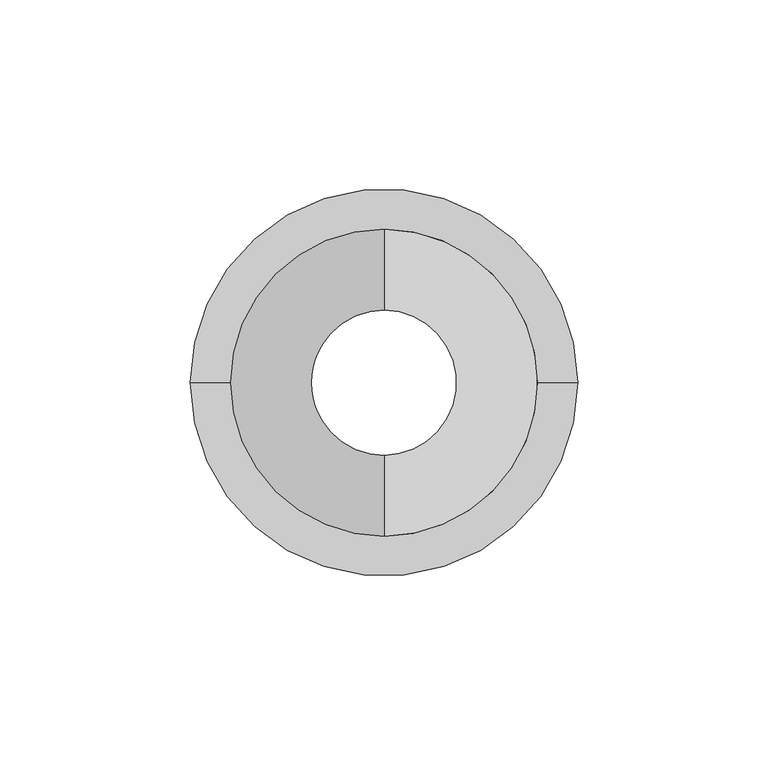
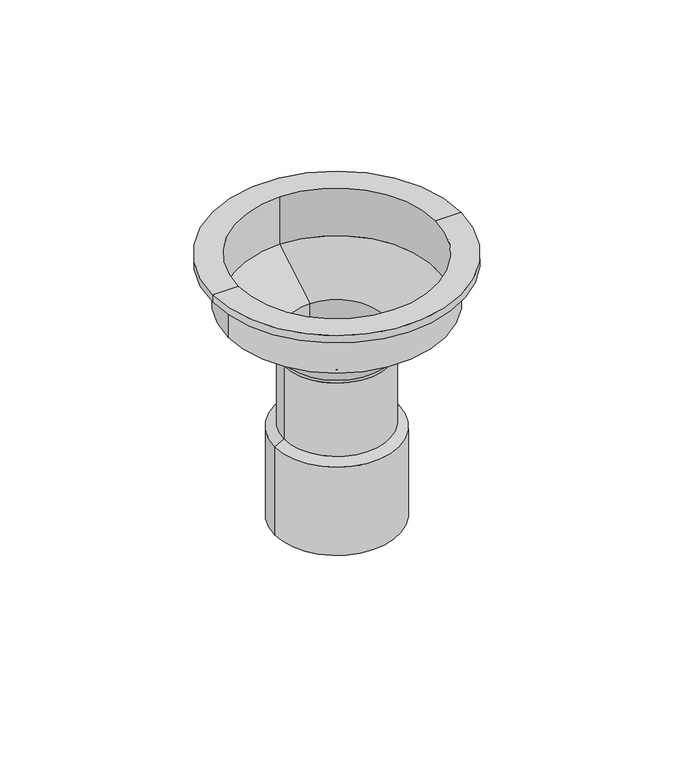
"""IFC4 building model written with IfcOpenShell, lengths in millimetres: proxy geometry, QF_BasketDrain_T&S Brass : QF_BasketDrain_T&S Brass."""

from ifc_helpers import new_model, si_unit, point, frame, origin, place, context, project, spatial, polyline, circle_curve, ellipse_curve, trimmed, source, transform, mapped, element, save
from ifc_brep_helpers import plane_surface, cylinder_surface, revolved_surface, advanced_brep


def specialty_equipment_44dcb793(model_context):
    return source(origin(), model_context, "Body", "AdvancedBrep", [
        advanced_brep(
        [(-25.4, -101.6, 449.2625), (25.4, -101.6, 449.2625), (19.05, -101.6, 449.2625), (0.0, -82.55, 449.2625), (-19.05, -101.6, 449.2625), (0.0, -120.65, 449.2625), (50.8, -101.6, 561.975), (-50.8, -101.6, 561.975), (-40.3518144, -101.6, 561.975), (0.0, -61.2481856, 561.975), (40.3518144, -101.6, 561.975), (0.0, -141.9518144, 561.975), (50.8, -101.6, 558.8), (-50.8, -101.6, 558.8), (44.45, -101.6, 558.8), (-44.45, -101.6, 558.8), (44.45, -101.6, 541.3375), (-44.45, -101.6, 541.3375), (22.253509, -101.6, 522.7124326), (-22.253509, -101.6, 522.7124326), (21.5046095, -101.6, 520.9369046), (-21.5046095, -101.6, 520.9369046), (21.5046095, -101.6, 489.3101953), (-21.5046095, -101.6, 489.3101953), (25.4, -101.6, 487.3625), (-25.4, -101.6, 487.3625), (0.0, -82.55, 528.6629098), (0.0, -120.65, 528.6629098), (0.0, -141.9518144, 541.3375), (0.0, -61.2481856, 541.3375)],
        [
            (0, 1, circle_curve(frame((0.0, -101.6, 449.2625), z_axis=(0.0, 0.0, -1.0), x_axis=(-1.0, 0.0, 0.0)), 25.4)),
            (1, 2),
            (2, 3, circle_curve(frame((0.0, -101.6, 449.2625), z_axis=(0.0, 0.0, 1.0), x_axis=(0.0, 1.0, 0.0)), 19.05)),
            (3, 4, circle_curve(frame((0.0, -101.6, 449.2625), z_axis=(0.0, 0.0, 1.0), x_axis=(0.0, 1.0, 0.0)), 19.05)),
            (4, 0),
            (1, 0, circle_curve(frame((0.0, -101.6, 449.2625), z_axis=(0.0, 0.0, -1.0), x_axis=(-1.0, 0.0, 0.0)), 25.4)),
            (4, 5, circle_curve(frame((0.0, -101.6, 449.2625), z_axis=(0.0, 0.0, 1.0), x_axis=(0.0, 1.0, 0.0)), 19.05)),
            (5, 2, circle_curve(frame((0.0, -101.6, 449.2625), z_axis=(0.0, 0.0, 1.0), x_axis=(0.0, 1.0, 0.0)), 19.05)),
            (6, 7, circle_curve(frame((0.0, -101.6, 561.975), z_axis=(0.0, 0.0, 1.0), x_axis=(-1.0, 0.0, 0.0)), 50.8)),
            (7, 8),
            (8, 9, circle_curve(frame((0.0, -101.6, 561.975), z_axis=(0.0, 0.0, -1.0), x_axis=(0.0, 1.0, 0.0)), 40.3518144)),
            (9, 10, circle_curve(frame((0.0, -101.6, 561.975), z_axis=(0.0, 0.0, -1.0), x_axis=(0.0, 1.0, 0.0)), 40.3518144)),
            (10, 6),
            (7, 6, circle_curve(frame((0.0, -101.6, 561.975), z_axis=(0.0, 0.0, 1.0), x_axis=(-1.0, 0.0, 0.0)), 50.8)),
            (10, 11, circle_curve(frame((0.0, -101.6, 561.975), z_axis=(0.0, 0.0, -1.0), x_axis=(0.0, 1.0, 0.0)), 40.3518144)),
            (11, 8, circle_curve(frame((0.0, -101.6, 561.975), z_axis=(0.0, 0.0, -1.0), x_axis=(0.0, 1.0, 0.0)), 40.3518144)),
            (6, 12),
            (12, 13, circle_curve(frame((0.0, -101.6, 558.8), z_axis=(0.0, 0.0, 1.0), x_axis=(-1.0, 0.0, 0.0)), 50.8)),
            (13, 7),
            (13, 12, circle_curve(frame((0.0, -101.6, 558.8), z_axis=(0.0, 0.0, 1.0), x_axis=(-1.0, 0.0, 0.0)), 50.8)),
            (12, 14),
            (14, 15, circle_curve(frame((0.0, -101.6, 558.8), z_axis=(0.0, 0.0, 1.0), x_axis=(-1.0, 0.0, 0.0)), 44.45)),
            (15, 13),
            (15, 14, circle_curve(frame((0.0, -101.6, 558.8), z_axis=(0.0, 0.0, 1.0), x_axis=(-1.0, 0.0, 0.0)), 44.45)),
            (14, 16),
            (16, 17, circle_curve(frame((0.0, -101.6, 541.3375), z_axis=(0.0, 0.0, 1.0), x_axis=(-1.0, 0.0, 0.0)), 44.45)),
            (17, 15),
            (17, 16, circle_curve(frame((0.0, -101.6, 541.3375), z_axis=(0.0, 0.0, 1.0), x_axis=(-1.0, 0.0, 0.0)), 44.45)),
            (16, 18, circle_curve(frame((61.3259975, -101.6, 498.6865616), z_axis=(0.0, -1.0, 0.0), x_axis=(-1.0, 0.0, 0.0)), 45.8683097)),
            (18, 19, circle_curve(frame((0.0, -101.6, 522.7124326), z_axis=(0.0, 0.0, 1.0), x_axis=(-1.0, 0.0, 0.0)), 22.253509)),
            (19, 17, circle_curve(frame((-61.3259975, -101.6, 498.6865616), z_axis=(0.0, -1.0, 0.0), x_axis=(1.0, 0.0, 0.0)), 45.8683097)),
            (19, 18, circle_curve(frame((0.0, -101.6, 522.7124326), z_axis=(0.0, 0.0, 1.0), x_axis=(-1.0, 0.0, 0.0)), 22.253509)),
            (18, 20),
            (20, 21, circle_curve(frame((0.0, -101.6, 520.9369046), z_axis=(0.0, 0.0, 1.0), x_axis=(-1.0, 0.0, 0.0)), 21.5046095)),
            (21, 19),
            (21, 20, circle_curve(frame((0.0, -101.6, 520.9369046), z_axis=(0.0, 0.0, 1.0), x_axis=(-1.0, 0.0, 0.0)), 21.5046095)),
            (20, 22),
            (22, 23, circle_curve(frame((0.0, -101.6, 489.3101953), z_axis=(0.0, 0.0, 1.0), x_axis=(-1.0, 0.0, 0.0)), 21.5046095)),
            (23, 21),
            (23, 22, circle_curve(frame((0.0, -101.6, 489.3101953), z_axis=(0.0, 0.0, 1.0), x_axis=(-1.0, 0.0, 0.0)), 21.5046095)),
            (22, 24),
            (24, 25, circle_curve(frame((0.0, -101.6, 487.3625), z_axis=(0.0, 0.0, 1.0), x_axis=(-1.0, 0.0, 0.0)), 25.4)),
            (25, 23),
            (25, 24, circle_curve(frame((0.0, -101.6, 487.3625), z_axis=(0.0, 0.0, 1.0), x_axis=(-1.0, 0.0, 0.0)), 25.4)),
            (0, 25),
            (24, 1),
            (26, 3),
            (5, 27),
            (27, 26, circle_curve(frame((0.0, -101.6, 528.6375), z_axis=(0.0, 0.0, 1.0), x_axis=(0.0, 1.0, 0.0)), 19.05)),
            (26, 27, circle_curve(frame((0.0, -101.6, 528.6375), z_axis=(0.0, 0.0, 1.0), x_axis=(0.0, 1.0, 0.0)), 19.05)),
            (28, 27),
            (26, 29),
            (29, 28, circle_curve(frame((0.0, -101.6, 541.3375), z_axis=(0.0, 0.0, 1.0), x_axis=(0.0, 1.0, 0.0)), 40.3518144)),
            (28, 29, circle_curve(frame((0.0, -101.6, 541.3375), z_axis=(0.0, 0.0, 1.0), x_axis=(0.0, 1.0, 0.0)), 40.3518144)),
            (29, 9),
            (11, 28),
        ],
        [
            plane_surface(frame((0.0, -101.6, 449.2625), z_axis=(0.0, 0.0, -1.0), x_axis=(-1.0, 0.0, 0.0))),
            plane_surface(frame((0.0, -101.6, 561.975), z_axis=(0.0, 0.0, 1.0), x_axis=(-1.0, 0.0, 0.0))),
            cylinder_surface(frame((0.0, -101.6, 449.2625), z_axis=(0.0, 0.0, -1.0), x_axis=(-1.0, 0.0, 0.0)), 50.8),
            plane_surface(frame((0.0, -101.6, 558.8), z_axis=(0.0, 0.0, -1.0), x_axis=(-1.0, 0.0, 0.0))),
            cylinder_surface(frame((0.0, -101.6, 449.2625), z_axis=(0.0, 0.0, -1.0), x_axis=(-1.0, 0.0, 0.0)), 44.45),
            revolved_surface(trimmed(ellipse_curve(frame((-61.3259975, -101.6, 498.6865616), z_axis=(0.0, 1.0, 0.0), x_axis=(1.0, 0.0, 0.0)), 45.8683097, 45.8683097), [point((-44.45, -101.6, 541.3375))], [point((-22.253509, -101.6, 522.7124326))], True, "CARTESIAN"), (0.0, -101.6, 449.2625), (0.0, 0.0, -1.0)),
            revolved_surface(polyline([(-22.253509, -101.6, 522.7124326), (-21.5046095, -101.6, 520.9369046)]), (0.0, -101.6, 449.2625), (0.0, 0.0, -1.0)),
            cylinder_surface(frame((0.0, -101.6, 449.2625), z_axis=(0.0, 0.0, -1.0), x_axis=(-1.0, 0.0, 0.0)), 21.5046095),
            revolved_surface(polyline([(-21.5046095, -101.6, 489.3101953), (-25.4, -101.6, 487.3625)]), (0.0, -101.6, 449.2625), (0.0, 0.0, -1.0)),
            cylinder_surface(frame((0.0, -101.6, 449.2625), z_axis=(0.0, 0.0, -1.0), x_axis=(-1.0, 0.0, 0.0)), 25.4),
            revolved_surface(polyline([(0.0, -82.55, 528.6629098), (0.0, -82.55, 449.2625)]), (0.0, -101.6, 449.2625), (0.0, 0.0, 1.0)),
            revolved_surface(polyline([(0.0, -61.2481856, 541.3375), (0.0, -82.55, 528.6375)]), (0.0, -101.6, 528.6375), (0.0, 0.0, 1.0)),
            revolved_surface(polyline([(0.0, -61.24818559999999, 561.975), (0.0, -61.24818559999999, 541.3375)]), (0.0, -101.6, 528.6375), (0.0, 0.0, 1.0)),
        ],
        [
            (0, [[1, 2, 3, 4, 5]]),
            (0, [[6, -5, 7, 8, -2]]),
            (1, [[9, 10, 11, 12, 13]]),
            (1, [[14, -13, 15, 16, -10]]),
            (2, [[-9, 17, 18, 19]]),
            (2, [[-14, -19, 20, -17]]),
            (3, [[-18, 21, 22, 23]]),
            (3, [[-20, -23, 24, -21]]),
            (4, [[-22, 25, 26, 27]]),
            (4, [[-24, -27, 28, -25]]),
            (5, [[-26, 29, 30, 31]]),
            (5, [[-28, -31, 32, -29]]),
            (6, [[-30, 33, 34, 35]]),
            (6, [[-32, -35, 36, -33]]),
            (7, [[-34, 37, 38, 39]]),
            (7, [[-36, -39, 40, -37]]),
            (8, [[-38, 41, 42, 43]]),
            (8, [[-40, -43, 44, -41]]),
            (9, [[-1, 45, -42, 46]]),
            (9, [[-6, -46, -44, -45]]),
            (10, [[47, -3, -8, 48, 49]]),
            (10, [[-47, 50, -48, -7, -4]]),
            (11, [[51, -50, 52, 53]]),
            (11, [[-51, 54, -52, -49]]),
            (12, [[-53, 55, -11, -16, 56]]),
            (12, [[-54, -56, -15, -12, -55]]),
        ],
    ),
    ])


if __name__ == "__main__":
    model = new_model("IFC4")
    model_context = context("Model", 3, world=origin())
    ifc_project = project(units=[si_unit("LENGTHUNIT", "METRE", prefix="MILLI")], contexts=[model_context])
    site = spatial("IfcSite", under=ifc_project)
    building = spatial("IfcBuilding", under=site)
    placement = place(None, origin())
    specialty_equipment_shape = specialty_equipment_44dcb793(model_context)
    element("IfcBuildingElementProxy", 1, Name="QF_BasketDrain_T&S Brass : QF_BasketDrain_T&S Brass", ObjectType="QF_BasketDrain_T&S Brass : QF_BasketDrain_T&S Brass", at=placement, inside=building, context=model_context, shape_type="MappedRepresentation", body=[
        mapped(specialty_equipment_shape, transform((0.0, 0.0, 0.0), x_axis=(1.0, 0.0, 0.0), y_axis=(0.0, 1.0, 0.0), z_axis=(0.0, 0.0, 1.0))),
    ])
    save(model, "model.ifc")

# Revit data of these elements
# Type "QF_BasketDrain_T&S Brass : QF_BasketDrain_T&S Brass"
#   Type Comments = "With Connected Overflow"
#   Manufacturer = "T & S Brass"
#   Description = "2\" lever Waste"
#   Sink Depth [instance default] = 2' - 1"
#   Overflow Centerline Height [instance default] = 0' - 8 1/2"
#   Indirect Waste Size = 2"
#   Indirect Waste Radius = 0' - 1"
#   Drain Height [instance default] = 1' - 10 3/16"
#   Drain Centerline FB [instance default] = 1' - 0 1/2"
#   Counter Height [instance default] = 2' - 8"
#   Basin Depth [instance default] = 0' - 10"
#   Material = QF_Finishes_Stainless Steel
#   Default Elevation = 0
#   Assembly Code = ""
# Element 1 (IfcBuildingElementProxy, "QF_BasketDrain_T&S Brass : QF_BasketDrain_T&S Brass")
#   Materials on its faces: "QF_Finishes_Stainless Steel"
# Materials
#   "QF_Finishes_Stainless Steel": class "Miscellaneous", colour RGB 189 187 185, transparency 0
